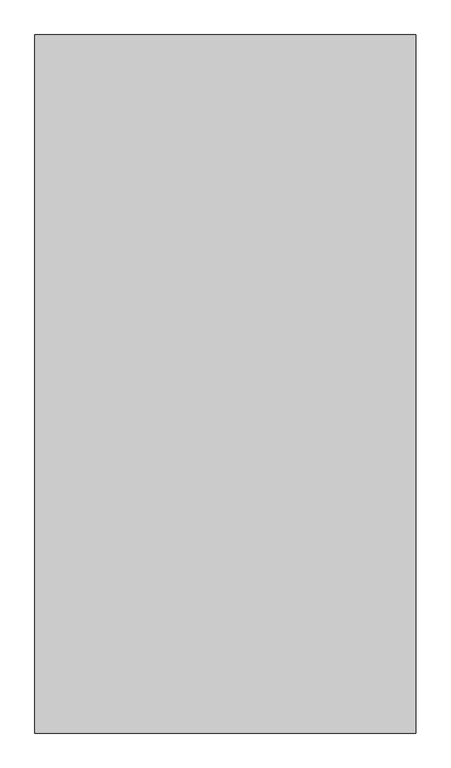
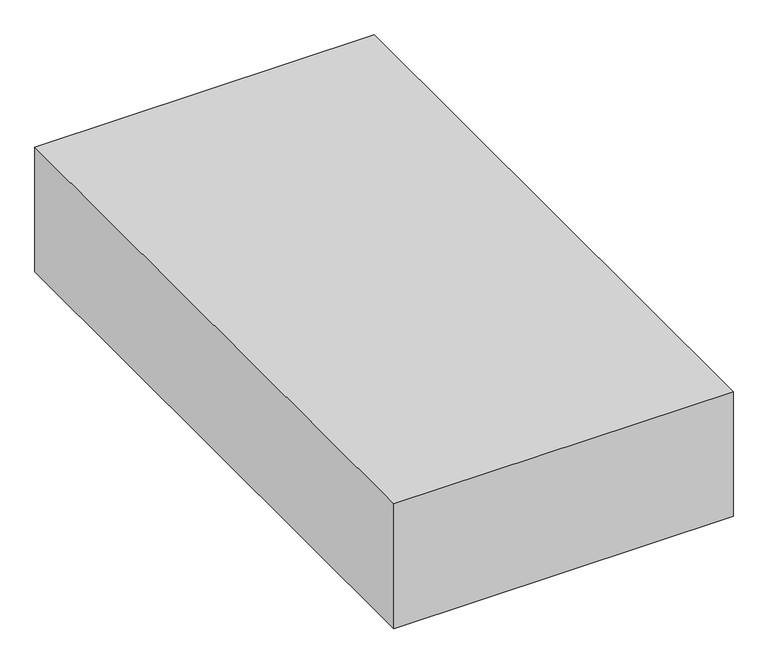
"""IFC4 building model written with IfcOpenShell, lengths in millimetres: proxy geometry, Space Planning Box_hec : Space Planning Box_hec."""

from ifc_helpers import new_model, si_unit, origin, origin_with_axes, place, context, project, spatial, polyline, outline, extrude, source, transform, mapped, element, save


def generic_models_f0561c1d(model_context):
    return source(origin(), model_context, "Body", "SweptSolid", [
        extrude(outline(polyline([(4500.0, 8250.0), (4500.0, -8250.0), (-4500.0, -8250.0), (-4500.0, 8250.0), (4500.0, 8250.0)])), origin_with_axes(), (0.0, 0.0, 1.0), 3500.0),
    ])


if __name__ == "__main__":
    model = new_model("IFC4")
    model_context = context("Model", 3, world=origin())
    ifc_project = project(units=[si_unit("LENGTHUNIT", "METRE", prefix="MILLI")], contexts=[model_context])
    site = spatial("IfcSite", under=ifc_project)
    building = spatial("IfcBuilding", under=site)
    placement = place(None, origin())
    generic_models_shape = generic_models_f0561c1d(model_context)
    element("IfcBuildingElementProxy", 1, Name="Space Planning Box_hec : Space Planning Box_hec", ObjectType="Space Planning Box_hec : Space Planning Box_hec", at=placement, inside=building, context=model_context, shape_type="MappedRepresentation", body=[
        mapped(generic_models_shape, transform((0.0, 0.0, 0.0), x_axis=(1.0, 0.0, 0.0), y_axis=(0.0, 1.0, 0.0), z_axis=(0.0, 0.0, 1.0))),
    ])
    save(model, "model.ifc")

# Revit data of these elements
# Type "Space Planning Box_hec : Space Planning Box_hec"
#   Type Comments = "..."
#   Room Name [instance default] = "?"
#   Interior Finish [instance default] = ""
#   Exterior Finish [instance default] = ""
#   Department [instance default] = ""
#   Assembly Code = "..."
#   ceiling height [instance default] = 0
#   Width [instance default] = 1524 mm
#   Program Area [instance default] = 0.00 m²
#   Length [instance default] = 1524 mm
#   Height [instance default] = 1524 mm
#   Area [instance default] = 2.32258 m²
#   Fill Color [instance default] = Cyan
#   Default Elevation = 0
# Element 1 (IfcBuildingElementProxy, "Space Planning Box_hec : Space Planning Box_hec")
#   Room Name = "Open Office"
#   Exterior Finish = "RF1..N/A,,EW1..N/A..N/A"
#   Department = "HV"
#   Width = 9000 mm
#   Program Area = 148.50 m²
#   Length = 16500 mm
#   Height = 3500 mm
#   Area = 148.50 m²
#   Fill Color = Lime
#   Materials on its faces: "Lime"
# Materials
#   "Cyan": class "Generic", colour RGB 0 255 255, transparency 0.2, Cost = 0
#   "Lime": class "Generic", colour RGB 0 255 0, transparency 0.2, Cost = 0
